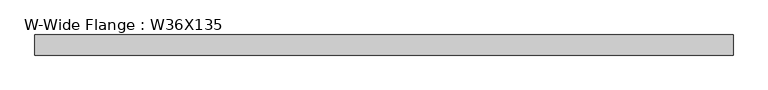
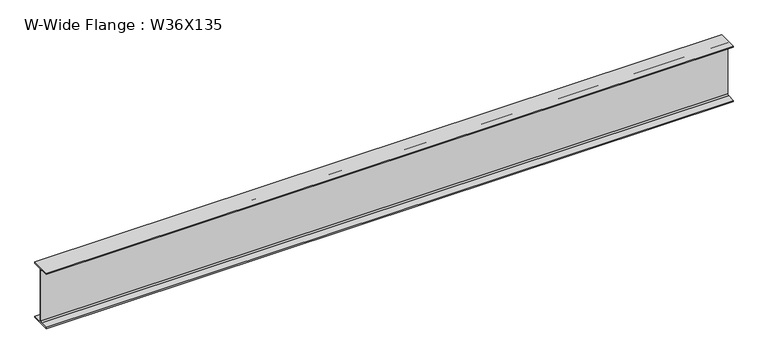
"""IFC4 building model written with IfcOpenShell, lengths in millimetres: beam geometry, W-Wide Flange : W36X135."""

from ifc_helpers import new_model, si_unit, point, frame, frame_2d, origin, place, context, project, spatial, polyline, circle_curve, trimmed, segment, composite_curve, outline, extrude, source, transform, mapped, element, save


def w_wide_flange_w36x135_edb61ff3(model_context):
    return source(origin(), model_context, "Body", "SweptSolid", [
        extrude(outline(composite_curve([segment(polyline([(152.4, -432.054), (152.4, -452.12), (-152.4, -452.12), (-152.4, -432.054), (-30.4165, -432.054)]), True, "CONTINUOUS"), segment(trimmed(circle_curve(frame_2d((-30.4165, -409.2575)), 22.7965), [point((-30.4165, -432.054))], [point((-7.62, -409.2575))], True, "CARTESIAN"), True, "CONTINUOUS"), segment(polyline([(-7.62, -409.2575), (-7.62, 409.2575)]), True, "CONTINUOUS"), segment(trimmed(circle_curve(frame_2d((-30.4165, 409.2575)), 22.7965), [point((-7.62, 409.2575))], [point((-30.4165, 432.054))], True, "CARTESIAN"), True, "CONTINUOUS"), segment(polyline([(-30.4165, 432.054), (-152.4, 432.054), (-152.4, 452.12), (152.4, 452.12), (152.4, 432.054), (30.4165, 432.054)]), True, "CONTINUOUS"), segment(trimmed(circle_curve(frame_2d((30.4165, 409.2575)), 22.7965), [point((30.4165, 432.054))], [point((7.62, 409.2575))], True, "CARTESIAN"), True, "CONTINUOUS"), segment(polyline([(7.62, 409.2575), (7.62, -409.2575)]), True, "CONTINUOUS"), segment(trimmed(circle_curve(frame_2d((30.4165, -409.2575)), 22.7965), [point((7.62, -409.2575))], [point((30.4165, -432.054))], True, "CARTESIAN"), True, "CONTINUOUS"), segment(polyline([(30.4165, -432.054), (152.4, -432.054)]), True, "CONTINUOUS")], self_intersect=False)), frame((-5233.2061528, 0.0, 0.0), z_axis=(1.0, 0.0, 0.0), x_axis=(0.0, 1.0, 0.0)), (0.0, 0.0, 1.0), 10580.7095618),
    ])


if __name__ == "__main__":
    model = new_model("IFC4")
    model_context = context("Model", 3, world=origin())
    ifc_project = project(units=[si_unit("LENGTHUNIT", "METRE", prefix="MILLI")], contexts=[model_context])
    site = spatial("IfcSite", under=ifc_project)
    building = spatial("IfcBuilding", under=site)
    placement = place(None, origin())
    w_wide_flange_w36x135_shape = w_wide_flange_w36x135_edb61ff3(model_context)
    element("IfcBeam", 1, ObjectType="W-Wide Flange : W36X135", at=placement, inside=building, context=model_context, shape_type="MappedRepresentation", body=[
        mapped(w_wide_flange_w36x135_shape, transform((0.0, 0.0, 0.0), x_axis=(1.0, 0.0, 0.0), y_axis=(0.0, 1.0, 0.0), z_axis=(0.0, 0.0, 1.0))),
    ])
    save(model, "model.ifc")

# Revit data of these elements
# Type "W-Wide Flange : W36X135"
#   Assembly Code = "B10"
#   W = 135
#   Length [instance default] = 1524 mm
#   bf = 304.8 mm
#   d = 904.24 mm
#   k = 42.863 mm
#   k2 = 22.797 mm
#   tf = 20.066 mm
#   tw = 15.24 mm
#   A = 0.0256129 m²
#   Structural Material [instance default] = Steel ASTM A992
# Element 1 (IfcBeam, "W-Wide Flange : W36X135")
#   Structural Material = Aluminum, Anodized Red
#   Materials on its faces: "Aluminum, Anodized Red"
# Materials
#   "Steel ASTM A992": class "Metal", colour RGB 128 0 0, transparency 0, Description = "Structural steel 50ksi", Cost = 0
#   "Aluminum, Anodized Red": class "Metal", colour RGB 120 120 120, transparency 0, Description = "Anodized aluminum, red", Cost = 0
